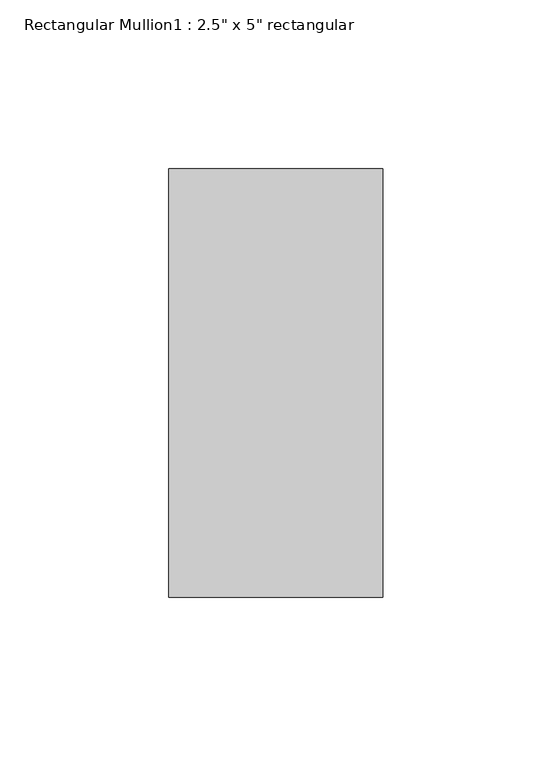
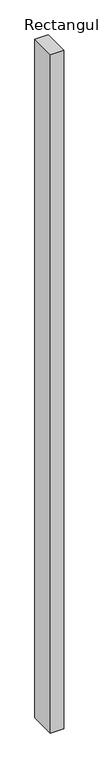
"""IFC4 building model written with IfcOpenShell, lengths in millimetres: member geometry."""

from ifc_helpers import new_model, si_unit, frame, origin, place, context, project, spatial, polyline, outline, extrude, source, transform, mapped, element, save


def member_74dafc5e(model_context):
    return source(origin(), model_context, "Body", "SweptSolid", [
        extrude(outline(polyline([(0.0, 63.5), (0.0, -63.5), (-63.5, -63.5), (-63.5, 63.5), (0.0, 63.5)])), frame((0.0, 0.0, -3414.1833333), z_axis=(0.0, 0.0, 1.0), x_axis=(1.0, 0.0, 0.0)), (0.0, 0.0, 1.0), 3414.1833333),
    ])


if __name__ == "__main__":
    model = new_model("IFC4")
    model_context = context("Model", 3, world=origin())
    ifc_project = project(units=[si_unit("LENGTHUNIT", "METRE", prefix="MILLI")], contexts=[model_context])
    site = spatial("IfcSite", under=ifc_project)
    building = spatial("IfcBuilding", under=site)
    placement = place(None, origin())
    member_shape = member_74dafc5e(model_context)
    element("IfcMember", 1, ObjectType="Rectangular Mullion1 : 2.5\" x 5\" rectangular", at=placement, inside=building, context=model_context, shape_type="MappedRepresentation", body=[
        mapped(member_shape, transform((0.0, 0.0, 0.0), x_axis=(1.0, 0.0, 0.0), y_axis=(0.0, 1.0, 0.0), z_axis=(0.0, 0.0, 1.0))),
    ])
    save(model, "model.ifc")

# Revit data of these elements
# Type "Rectangular Mullion1 : 2.5\" x 5\" rectangular"
#   built-in parameter 1007304 = 0.416667 (stored number, unit not read)
#   built-in parameter 1007301 = 0.104167 (stored number, unit not read)
#   built-in parameter 1007300 = 0.104167 (stored number, unit not read)
# Element 1 (IfcMember, "Rectangular Mullion1 : 2.5\" x 5\" rectangular")
#   Materials on its faces: "support-frame"
# Materials
#   "support-frame": class "Unassigned", colour RGB 233 233 233, transparency 0, Cost = 0
